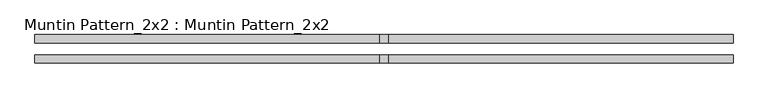
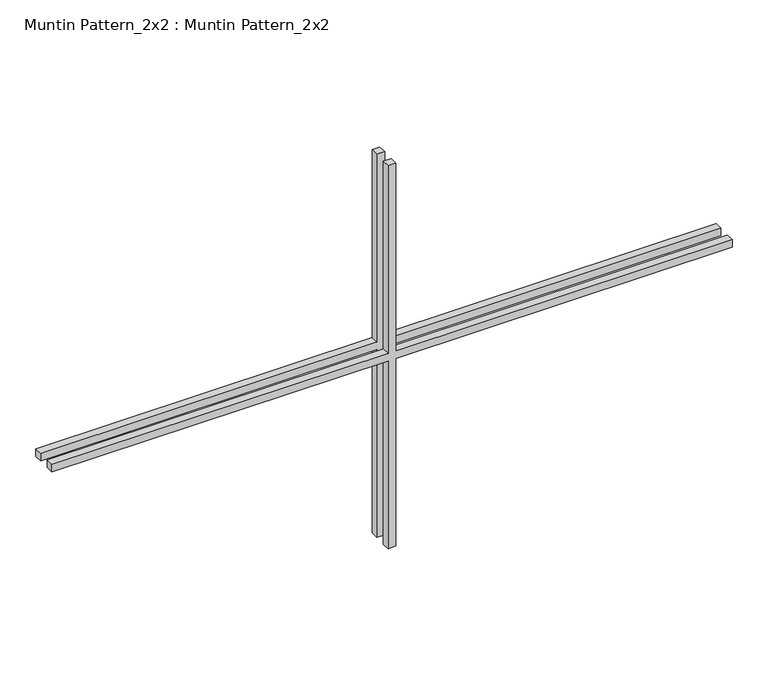
"""IFC4 building model written with IfcOpenShell, lengths in millimetres: proxy geometry, Muntin Pattern_2x2 : Muntin Pattern_2x2."""

from ifc_helpers import new_model, si_unit, frame, origin, place, context, project, spatial, polyline, outline, extrude, source, transform, mapped, element, save


def muntin_pattern_2x2_muntin_pattern_2x2_d2a59152(model_context):
    return source(origin(), model_context, "Body", "SweptSolid", [
        extrude(outline(polyline([(331.7875, -6.35), (331.7875, -546.1), (319.0875, -546.1), (319.0875, -6.35), (0.0, -6.35), (0.0, 6.35), (319.0875, 6.35), (319.0875, 546.1), (331.7875, 546.1), (331.7875, 6.35), (650.875, 6.35), (650.875, -6.35), (331.7875, -6.35)])), frame((0.0, -22.225, 0.0), z_axis=(0.0, 1.0, 0.0), x_axis=(0.0, 0.0, 1.0)), (0.0, 0.0, 1.0), 12.7),
        extrude(outline(polyline([(331.7875, -6.35), (331.7875, -546.1), (319.0875, -546.1), (319.0875, -6.35), (0.0, -6.35), (0.0, 6.35), (319.0875, 6.35), (319.0875, 546.1), (331.7875, 546.1), (331.7875, 6.35), (650.875, 6.35), (650.875, -6.35), (331.7875, -6.35)])), frame((0.0, 9.525, 0.0), z_axis=(0.0, 1.0, 0.0), x_axis=(0.0, 0.0, 1.0)), (0.0, 0.0, 1.0), 12.7),
    ])


if __name__ == "__main__":
    model = new_model("IFC4")
    model_context = context("Model", 3, world=origin())
    ifc_project = project(units=[si_unit("LENGTHUNIT", "METRE", prefix="MILLI")], contexts=[model_context])
    site = spatial("IfcSite", under=ifc_project)
    building = spatial("IfcBuilding", under=site)
    placement = place(None, origin())
    muntin_pattern_2x2_muntin_pattern_2x2_shape = muntin_pattern_2x2_muntin_pattern_2x2_d2a59152(model_context)
    element("IfcBuildingElementProxy", 1, Name="Muntin Pattern_2x2 : Muntin Pattern_2x2", ObjectType="Muntin Pattern_2x2 : Muntin Pattern_2x2", at=placement, inside=building, context=model_context, shape_type="MappedRepresentation", body=[
        mapped(muntin_pattern_2x2_muntin_pattern_2x2_shape, transform((0.0, 0.0, 0.0), x_axis=(1.0, 0.0, 0.0), y_axis=(0.0, 1.0, 0.0), z_axis=(0.0, 0.0, 1.0))),
    ])
    save(model, "model.ifc")

# Revit data of these elements
# Type "Muntin Pattern_2x2 : Muntin Pattern_2x2"
#   Width [instance default] = 4' - 0"
#   Thickness = 0' - 0 1/2"
#   Height [instance default] = 4' - 0"
#   Distance = 0' - 0 3/4"
#   Interior Material [instance default] = none
#   Exterior Material [instance default] = none
# Element 1 (IfcBuildingElementProxy, "Muntin Pattern_2x2 : Muntin Pattern_2x2")
#   Width = 3' - 7"
#   Height = 2' - 1 5/8"
#   Interior Material = Wood - Stained
#   Exterior Material = Clad - White
#   Materials on its faces: "Clad - White", "Wood - Stained"
# Materials
#   "Clad - White": class "Wood", colour RGB 242 242 238, transparency 0, Cost = 0
#   "Wood - Stained": class "Wood", colour RGB 224 178 126, transparency 0, Cost = 0
